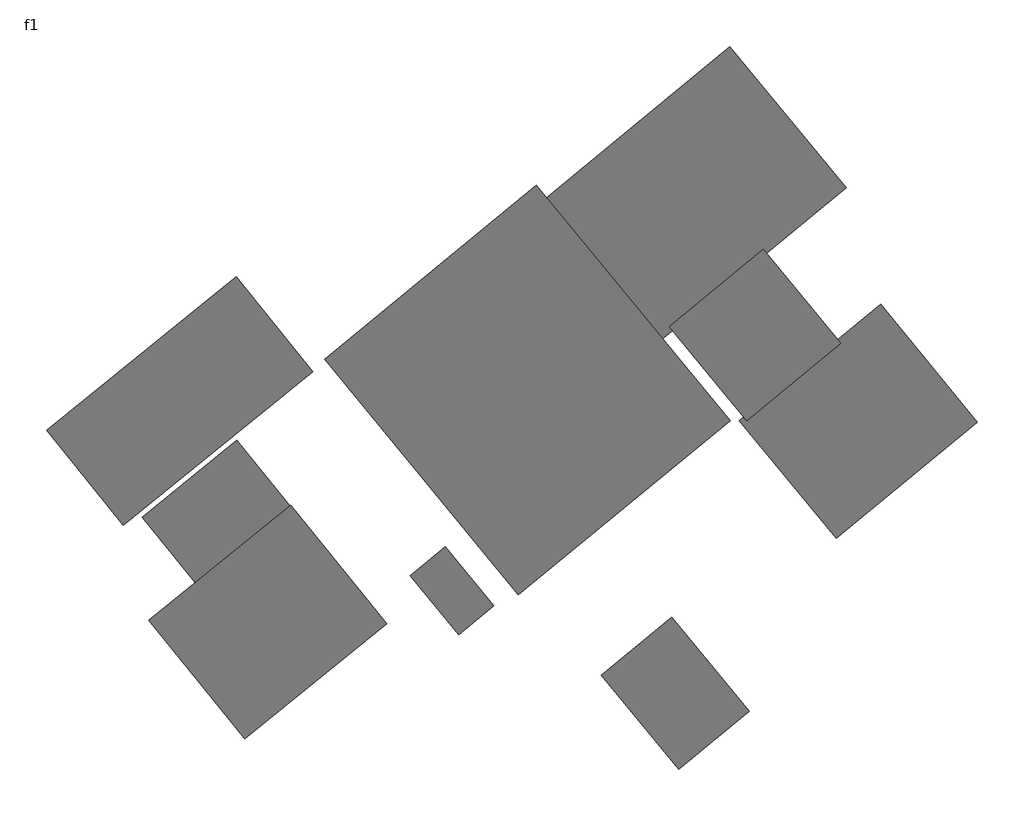
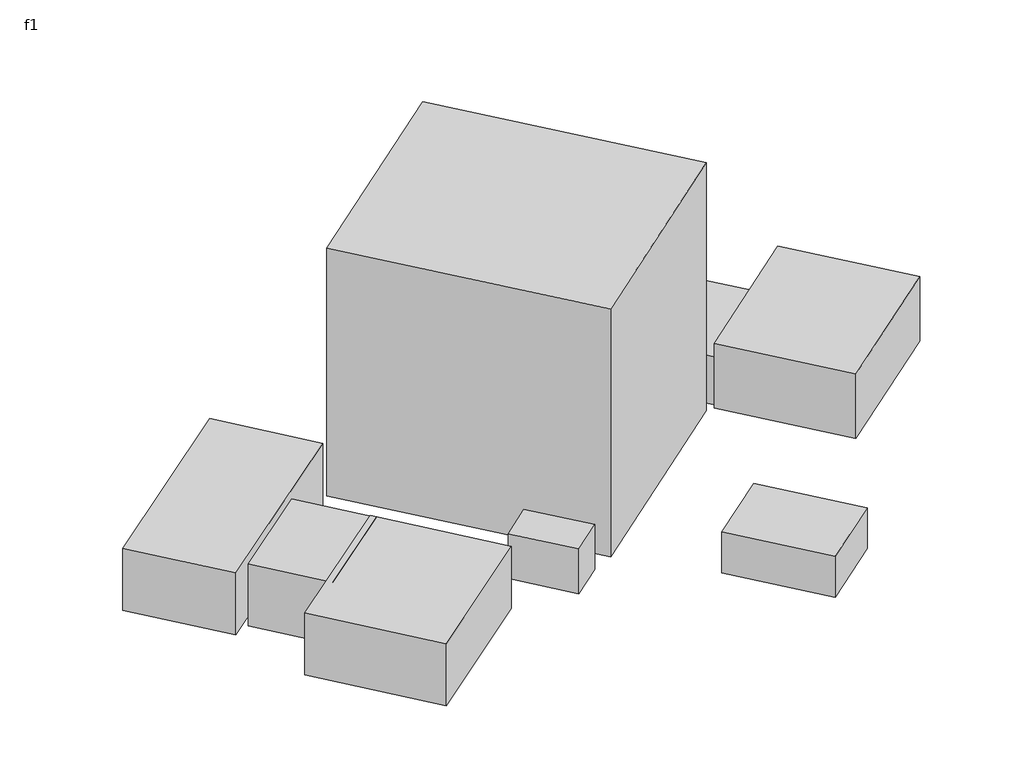
# One storey: 11 proxies.
"""IFC4 building model written with IfcOpenShell, lengths in millimetres."""

from ifc_helpers import new_model, si_unit, frame, origin, place, context, project, spatial, polyline, outline, extrude, element, save

model = new_model("IFC4")

# Units and contexts
model_context = context("Model", 3, world=origin())
ifc_project = project(units=[si_unit("LENGTHUNIT", "METRE", prefix="MILLI")], contexts=[model_context])

# Site, building, storey
site = spatial("IfcSite", under=ifc_project)
building = spatial("IfcBuilding", under=site)
storey = spatial("IfcBuildingStorey", under=building, Name="f1", Elevation=3100.0)

# Proxies
placement = place(None, origin())
element("IfcBuildingElementProxy", 1, Name="公共-开敞 : Visitor Screening/Bag Check", ObjectType="公共-开敞 : Visitor Screening/Bag Check", at=placement, inside=storey, context=model_context, shape_type="SweptSolid", body=[
    extrude(outline(polyline([(-12238.208834, 13312.6525372), (-18455.3765257, 8278.0894088), (-26007.2212183, 17603.8409463), (-19790.0535266, 22638.4040747), (-12238.208834, 13312.6525372)])), frame((0.0, 0.0, 3100.0), z_axis=(0.0, 0.0, 1.0), x_axis=(1.0, 0.0, 0.0)), (0.0, 0.0, 1.0), 6000.0),
])
element("IfcBuildingElementProxy", 2, Name="公共-开敞 : Ticketing and Information Desk", ObjectType="公共-开敞 : Ticketing and Information Desk", at=placement, inside=storey, context=model_context, shape_type="SweptSolid", body=[
    extrude(outline(polyline([(-20945.8073222, 16199.6559889), (-17857.1841291, 18741.389014), (-14680.0178477, 14880.6100226), (-17768.6410408, 12338.8769975), (-20945.8073222, 16199.6559889)])), frame((0.0, 0.0, 3100.0), z_axis=(0.0, 0.0, 1.0), x_axis=(1.0, 0.0, 0.0)), (0.0, 0.0, 1.0), 6000.0),
])
element("IfcBuildingElementProxy", 3, Name="公共-开敞 : Café/Bar", ObjectType="公共-开敞 : Café/Bar", at=placement, inside=storey, context=model_context, shape_type="SweptSolid", body=[
    extrude(outline(polyline([(-12058.197654, 13973.909269), (-19683.3967294, 23239.7788482), (-7328.903957, 33406.7109488), (296.2951184, 24140.8413695), (-12058.197654, 13973.909269)])), frame((0.0, 0.0, 3100.0), z_axis=(0.0, 0.0, 1.0), x_axis=(1.0, 0.0, 0.0)), (0.0, 0.0, 1.0), 5000.0),
])
element("IfcBuildingElementProxy", 4, Name="公共-开敞 : Formal Restaurant", ObjectType="公共-开敞 : Formal Restaurant", at=placement, inside=storey, context=model_context, shape_type="SweptSolid", body=[
    extrude(outline(polyline([(-355.8322971, 1147.2606983), (-6710.16486, 8868.8186811), (2555.7047193, 16494.0177565), (8910.0372821, 8772.4597737), (-355.8322971, 1147.2606983)])), frame((0.0, 0.0, 3100.0), z_axis=(0.0, 0.0, 1.0), x_axis=(1.0, 0.0, 0.0)), (0.0, 0.0, 1.0), 5200.0),
])
element("IfcBuildingElementProxy", 5, Name="公共-开敞 : lobby Café/Bar", ObjectType="公共-开敞 : lobby Café/Bar", at=placement, inside=storey, context=model_context, shape_type="SweptSolid", body=[
    extrude(outline(polyline([(-5142.2144043, 20114.3454078), (-58.748354, 13937.0990216), (-6235.9947402, 8853.6329713), (-11319.4607905, 15030.8793575), (-5142.2144043, 20114.3454078)])), frame((0.0, 0.0, 3100.0), z_axis=(0.0, 0.0, 1.0), x_axis=(1.0, 0.0, 0.0)), (0.0, 0.0, 1.0), 3900.0),
])
element("IfcBuildingElementProxy", 6, Name="公共-开敞 : lobby Formal Restaurant", ObjectType="公共-开敞 : lobby Formal Restaurant", at=placement, inside=storey, context=model_context, shape_type="SweptSolid", body=[
    extrude(outline(polyline([(-28298.4201975, -1318.5492601), (-25981.9528027, 587.7505087), (-22804.7865213, -3273.0284826), (-25121.2539161, -5179.3282515), (-28298.4201975, -1318.5492601)])), frame((0.0, 0.0, 3100.0), z_axis=(0.0, 0.0, 1.0), x_axis=(1.0, 0.0, 0.0)), (0.0, 0.0, 1.0), 3600.0),
])
element("IfcBuildingElementProxy", 7, Name="公共-开敞 : Design Store", ObjectType="公共-开敞 : Design Store", at=placement, inside=storey, context=model_context, shape_type="SweptSolid", body=[
    extrude(outline(polyline([(-36127.4685132, 3334.407767), (-29834.2646027, -4437.0518475), (-39160.0161402, -11988.8965401), (-45453.2200507, -4217.4369256), (-36127.4685132, 3334.407767)])), frame((0.0, 0.0, 3100.0), z_axis=(0.0, 0.0, 1.0), x_axis=(1.0, 0.0, 0.0)), (0.0, 0.0, 1.0), 5000.0),
])
element("IfcBuildingElementProxy", 8, Name="公共-开敞 : Lobby-Atrium", ObjectType="公共-开敞 : Lobby-Atrium", at=placement, inside=storey, context=model_context, shape_type="SweptSolid", body=[
    extrude(outline(polyline([(-20013.9394498, 24318.8457243), (-7305.2743241, 8875.7297588), (-21204.078693, -2562.0688543), (-33912.7438187, 12881.0471111), (-20013.9394498, 24318.8457243)])), frame((0.0, 0.0, 3100.0), z_axis=(0.0, 0.0, 1.0), x_axis=(1.0, 0.0, 0.0)), (0.0, 0.0, 1.0), 20000.0),
])
element("IfcBuildingElementProxy", 9, Name="公共-开敞 : Museum Store", ObjectType="公共-开敞 : Museum Store", at=placement, inside=storey, context=model_context, shape_type="SweptSolid", body=[
    extrude(outline(polyline([(-39714.3199437, 18301.1887854), (-34679.7568153, 12084.0210938), (-47114.0921986, 2014.894837), (-52148.655327, 8232.0625286), (-39714.3199437, 18301.1887854)])), frame((0.0, 0.0, 3100.0), z_axis=(0.0, 0.0, 1.0), x_axis=(1.0, 0.0, 0.0)), (0.0, 0.0, 1.0), 5000.0),
])
element("IfcBuildingElementProxy", 10, Name="临时私有-封闭 : Restrooms-Gallery-1f", ObjectType="临时私有-封闭 : Restrooms-Gallery-1f", at=placement, inside=storey, context=model_context, shape_type="SweptSolid", body=[
    extrude(outline(polyline([(-6052.7890456, -10193.6386218), (-10685.7238352, -14006.2381595), (-15769.1898855, -7828.9917733), (-11136.2550959, -4016.3922356), (-6052.7890456, -10193.6386218)])), frame((0.0, 0.0, 3100.0), z_axis=(0.0, 0.0, 1.0), x_axis=(1.0, 0.0, 0.0)), (0.0, 0.0, 1.0), 3300.0),
])
element("IfcBuildingElementProxy", 11, Name="公共-开敞 : Stock Room and Offices", ObjectType="公共-开敞 : Stock Room and Offices", at=placement, inside=storey, context=model_context, shape_type="SweptSolid", body=[
    extrude(outline(polyline([(-42102.4996768, -2115.8724169), (-45878.4220231, 2547.0033518), (-39661.2543314, 7581.5664802), (-35885.3319851, 2918.6907115), (-42102.4996768, -2115.8724169)])), frame((0.0, 0.0, 3100.0), z_axis=(0.0, 0.0, 1.0), x_axis=(1.0, 0.0, 0.0)), (0.0, 0.0, 1.0), 5000.0),
])

save(model, "model.ifc")

# Revit data of these elements
# Type "公共-开敞 : Visitor Screening/Bag Check"
#   Default Elevation = 1219.2 mm
#   半临时私有(开敞)_空间_层高 = 1440 mm
#   公共_开敞_房间_面积 = 96.00 m²
#   公共_开敞_房间_进深 = 8000 mm
#   公共_开敞_房间_开间 = 12000 mm
#   公共_开敞_房间_层高 = 6000 mm
# Type "公共-开敞 : Ticketing and Information Desk"
#   Default Elevation = 1219.2 mm
#   半临时私有(开敞)_空间_层高 = 1440 mm
#   公共_开敞_房间_面积 = 20.00 m²
#   公共_开敞_房间_进深 = 4000 mm
#   公共_开敞_房间_开间 = 5000 mm
#   公共_开敞_房间_层高 = 6000 mm
# Type "公共-开敞 : Café/Bar"
#   Default Elevation = 1219.2 mm
#   半临时私有(开敞)_空间_层高 = 1440 mm
#   公共_开敞_房间_面积 = 192.00 m²
#   公共_开敞_房间_进深 = 12000 mm
#   公共_开敞_房间_开间 = 16000 mm
#   公共_开敞_房间_层高 = 5000 mm
# Type "公共-开敞 : Formal Restaurant"
#   Default Elevation = 1219.2 mm
#   半临时私有(开敞)_空间_层高 = 1440 mm
#   公共_开敞_房间_面积 = 120.00 m²
#   公共_开敞_房间_进深 = 10000 mm
#   公共_开敞_房间_开间 = 12000 mm
#   公共_开敞_房间_层高 = 5200 mm
# Type "公共-开敞 : lobby Café/Bar"
#   Default Elevation = 1219.2 mm
#   半临时私有(开敞)_空间_层高 = 1440 mm
#   公共_开敞_房间_面积 = 64.00 m²
#   公共_开敞_房间_进深 = 8000 mm
#   公共_开敞_房间_开间 = 8000 mm
#   公共_开敞_房间_层高 = 3900 mm
# Type "公共-开敞 : lobby Formal Restaurant"
#   Default Elevation = 1219.2 mm
#   半临时私有(开敞)_空间_层高 = 1440 mm
#   公共_开敞_房间_面积 = 15.00 m²
#   公共_开敞_房间_进深 = 3000 mm
#   公共_开敞_房间_开间 = 5000 mm
#   公共_开敞_房间_层高 = 3600 mm
# Type "公共-开敞 : Design Store"
#   Default Elevation = 1219.2 mm
#   半临时私有(开敞)_空间_层高 = 1440 mm
#   公共_开敞_房间_面积 = 120.00 m²
#   公共_开敞_房间_进深 = 10000 mm
#   公共_开敞_房间_开间 = 12000 mm
#   公共_开敞_房间_层高 = 5000 mm
# Type "公共-开敞 : Lobby-Atrium"
#   Default Elevation = 1219.2 mm
#   半临时私有(开敞)_空间_层高 = 1440 mm
#   公共_开敞_房间_面积 = 360.00 m²
#   公共_开敞_房间_进深 = 20000 mm
#   公共_开敞_房间_开间 = 18000 mm
#   公共_开敞_房间_层高 = 20000 mm
# Type "公共-开敞 : Museum Store"
#   Default Elevation = 1219.2 mm
#   半临时私有(开敞)_空间_层高 = 1440 mm
#   公共_开敞_房间_面积 = 128.00 m²
#   公共_开敞_房间_进深 = 8000 mm
#   公共_开敞_房间_开间 = 16000 mm
#   公共_开敞_房间_层高 = 5000 mm
# Type "临时私有-封闭 : Restrooms-Gallery-1f"
#   Default Elevation = 1219.2 mm
#   临时私有_封闭_房间_面积 = 48.00 m²
#   临时私有_封闭_房间_进深 = 6000 mm
#   临时私有_封闭_房间_开间 = 8000 mm
#   临时私有_封闭_房间_层高 = 3300 mm
# Type "公共-开敞 : Stock Room and Offices"
#   Default Elevation = 1219.2 mm
#   半临时私有(开敞)_空间_层高 = 1440 mm
#   公共_开敞_房间_面积 = 48.00 m²
#   公共_开敞_房间_进深 = 6000 mm
#   公共_开敞_房间_开间 = 8000 mm
#   公共_开敞_房间_层高 = 5000 mm
# Element 1 (IfcBuildingElementProxy, "公共-开敞 : Visitor Screening/Bag Check")
#   Phase Created = 新构造
#   Materials on its faces: "公共_开敞_房间"
# Element 2 (IfcBuildingElementProxy, "公共-开敞 : Ticketing and Information Desk")
#   Phase Created = 新构造
#   Materials on its faces: "公共_开敞_房间"
# Element 3 (IfcBuildingElementProxy, "公共-开敞 : Café/Bar")
#   Phase Created = 新构造
#   Materials on its faces: "公共_开敞_房间"
# Element 4 (IfcBuildingElementProxy, "公共-开敞 : Formal Restaurant")
#   Phase Created = 新构造
#   Materials on its faces: "公共_开敞_房间"
# Element 5 (IfcBuildingElementProxy, "公共-开敞 : lobby Café/Bar")
#   Phase Created = 新构造
#   Materials on its faces: "公共_开敞_房间"
# Element 6 (IfcBuildingElementProxy, "公共-开敞 : lobby Formal Restaurant")
#   Phase Created = 新构造
#   Materials on its faces: "公共_开敞_房间"
# Element 7 (IfcBuildingElementProxy, "公共-开敞 : Design Store")
#   Phase Created = 新构造
#   Materials on its faces: "公共_开敞_房间"
# Element 8 (IfcBuildingElementProxy, "公共-开敞 : Lobby-Atrium")
#   Phase Created = 新构造
#   Materials on its faces: "公共_开敞_房间"
# Element 9 (IfcBuildingElementProxy, "公共-开敞 : Museum Store")
#   Phase Created = 新构造
#   Materials on its faces: "公共_开敞_房间"
# Element 10 (IfcBuildingElementProxy, "临时私有-封闭 : Restrooms-Gallery-1f")
#   Phase Created = 新构造
#   Materials on its faces: "临时私有_封闭_房间"
# Element 11 (IfcBuildingElementProxy, "公共-开敞 : Stock Room and Offices")
#   Phase Created = 新构造
#   Materials on its faces: "公共_开敞_房间"
# Materials
#   "公共_开敞_房间": class "玻璃", colour RGB 255 255 255, transparency 0
#   "临时私有_封闭_房间": class "其他", colour RGB 77 38 0, transparency 0
